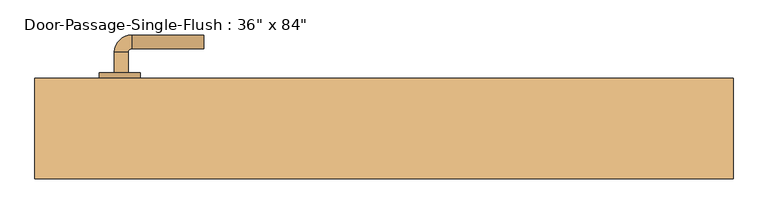
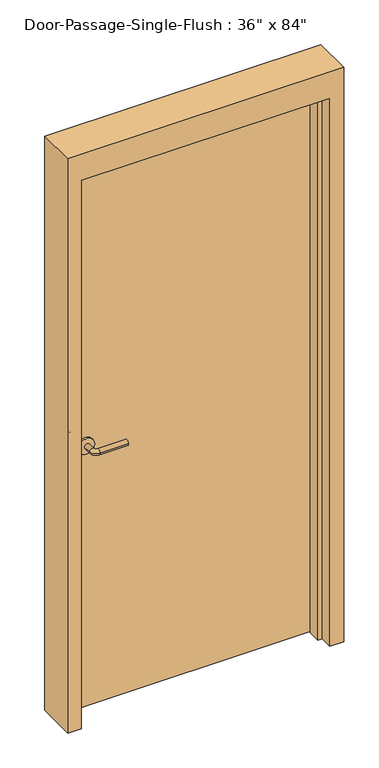
"""IFC4 building model written with IfcOpenShell, lengths in millimetres: door geometry."""

import ifcopenshell
import ifcopenshell.guid

model = None  # the IFC model being written
_history = None  # IfcOwnerHistory: only IFC2X3 demands one
_inside = {}  # id of a spatial element -> (the spatial element, [elements in it])
_under = {}  # id of a project, library or spatial element -> (it, [spatial elements below it])
_declared = {}  # id of a project -> (the project, [libraries it declares])
_typed = {}  # id of a type object -> (the type object, [elements of that type])
_made_of = {}  # id of a material, layer set ... -> (it, [elements and type objects made of it])


def new_model(schema):
    """Start an empty IFC model of exactly this schema.

    Asked for "IFC4X3", IfcOpenShell would pick the latest addendum, in which some entities
    have other attributes; the version numbers below select the first issue.
    IFC2X3 requires an IfcOwnerHistory on every rooted entity: one is made here for all.
    """
    global model, _history
    if schema == "IFC4X3":
        model = ifcopenshell.file(schema_version=(4, 3, 0, 0))
    else:
        model = ifcopenshell.file(schema=schema)
    _inside.clear()
    _under.clear()
    _declared.clear()
    _typed.clear()
    _made_of.clear()
    _history = None
    if model.schema == "IFC2X3":
        org = make("IfcOrganization", Name="unknown")
        user = make(
            "IfcPersonAndOrganization",
            ThePerson=make("IfcPerson", FamilyName="unknown"),
            TheOrganization=org,
        )
        app = make(
            "IfcApplication",
            ApplicationDeveloper=org,
            Version="unknown",
            ApplicationFullName="unknown",
            ApplicationIdentifier="unknown",
        )
        _history = make(
            "IfcOwnerHistory",
            OwningUser=user,
            OwningApplication=app,
            ChangeAction="ADDED",
            CreationDate=0,
        )
    return model


def make(cls, **values):
    """One entity of the class cls with the attributes given. An attribute that is None is left unset."""
    return model.create_entity(
        cls, **{name: value for name, value in values.items() if value is not None}
    )


def rooted(cls, **values):
    """An entity with a GlobalId (a new one), such as an element, a storey or a relation."""
    return make(cls, GlobalId=ifcopenshell.guid.new(), OwnerHistory=_history, **values)


def si_unit(unit_type, name, prefix=None):
    """IfcSIUnit, for example si_unit("LENGTHUNIT", "METRE", prefix="MILLI")."""
    return make("IfcSIUnit", UnitType=unit_type, Prefix=prefix, Name=name)


def assignment(units):
    """IfcUnitAssignment: the units of a project."""
    return None if units is None else make("IfcUnitAssignment", Units=units)


def point(xyz):
    """IfcCartesianPoint."""
    return None if xyz is None else make("IfcCartesianPoint", Coordinates=xyz)


def direction(xyz):
    """IfcDirection."""
    return None if xyz is None else make("IfcDirection", DirectionRatios=xyz)


def frame(location, z_axis=None, x_axis=None):
    """IfcAxis2Placement3D, a coordinate frame: its origin and axes. An axis left out is left unset."""
    return make(
        "IfcAxis2Placement3D",
        Location=point(location),
        Axis=direction(z_axis),
        RefDirection=direction(x_axis),
    )


def frame_2d(location, x_axis=None):
    """IfcAxis2Placement2D, a coordinate frame in the plane: its origin and x axis."""
    return make(
        "IfcAxis2Placement2D", Location=point(location), RefDirection=direction(x_axis)
    )


def origin():
    """The frame at (0, 0, 0) with its axes left unset."""
    return frame((0.0, 0.0, 0.0))


def origin_with_axes():
    """The frame at (0, 0, 0) with the z axis (0, 0, 1) and the x axis (1, 0, 0) written out."""
    return frame((0.0, 0.0, 0.0), z_axis=(0.0, 0.0, 1.0), x_axis=(1.0, 0.0, 0.0))


def place(relative_to, where):
    """IfcLocalPlacement: puts the frame where relative to a parent placement (None: the world)."""
    return make(
        "IfcLocalPlacement", PlacementRelTo=relative_to, RelativePlacement=where
    )


def context(
    kind, dimensions, precision=None, world=None, true_north=None, identifier=None
):
    """IfcGeometricRepresentationContext, for example the 3D "Model" context."""
    return make(
        "IfcGeometricRepresentationContext",
        ContextIdentifier=identifier,
        ContextType=kind,
        CoordinateSpaceDimension=dimensions,
        Precision=precision,
        WorldCoordinateSystem=world,
        TrueNorth=true_north,
    )


def project(units=None, contexts=None):
    """IfcProject with its units and contexts."""
    return rooted(
        "IfcProject",
        Name="project",
        RepresentationContexts=contexts,
        UnitsInContext=assignment(units),
    )


def spatial(cls, under=None, at=None, **own):
    """A site, building, storey or space (cls), placed at a placement, below another one or the project."""
    s = rooted(cls, ObjectPlacement=at, **own)
    if under is not None:
        _under.setdefault(under.id(), (under, []))[1].append(s)
    return s


def polyline(points):
    """IfcPolyline through the points."""
    return make("IfcPolyline", Points=[point(p) for p in points])


def circle_curve(where, radius):
    """IfcCircle in the frame where."""
    return make("IfcCircle", Position=where, Radius=radius)


def ellipse_curve(where, semi_axis1, semi_axis2):
    """IfcEllipse in the frame where."""
    return make(
        "IfcEllipse", Position=where, SemiAxis1=semi_axis1, SemiAxis2=semi_axis2
    )


def trimmed(basis, trim1, trim2, sense, master):
    """IfcTrimmedCurve: the piece of a basis curve between two trims."""
    return make(
        "IfcTrimmedCurve",
        BasisCurve=basis,
        Trim1=trim1,
        Trim2=trim2,
        SenseAgreement=sense,
        MasterRepresentation=master,
    )


def segment(curve, same_sense, transition):
    """IfcCompositeCurveSegment."""
    return make(
        "IfcCompositeCurveSegment",
        Transition=transition,
        SameSense=same_sense,
        ParentCurve=curve,
    )


def composite_curve(segments, self_intersect=None):
    """IfcCompositeCurve: segments joined end to end."""
    return make("IfcCompositeCurve", Segments=segments, SelfIntersect=self_intersect)


def outline(outer, holes=None, kind="AREA"):
    """IfcArbitraryClosedProfileDef: a profile drawn as a closed curve; with holes, ...WithVoids."""
    if holes is None:
        return make("IfcArbitraryClosedProfileDef", ProfileType=kind, OuterCurve=outer)
    return make(
        "IfcArbitraryProfileDefWithVoids",
        ProfileType=kind,
        OuterCurve=outer,
        InnerCurves=holes,
    )


def extrude(swept, where, along, depth):
    """IfcExtrudedAreaSolid: the profile swept, set in the frame where, extruded along a direction by depth."""
    return make(
        "IfcExtrudedAreaSolid",
        SweptArea=swept,
        Position=where,
        ExtrudedDirection=direction(along),
        Depth=depth,
    )


def faces_of(points, faces, orient=None, outer=None):
    """IfcFace entities. A face is a list of loops; a loop is a list of indices into points, from 0.

    orient and outer hold one flag for each loop. By default every Orientation is true, the
    first loop of a face is its IfcFaceOuterBound and the others are IfcFaceBound.
    """
    made = []
    for i, loops in enumerate(faces):
        bounds = []
        for j, loop in enumerate(loops):
            is_outer = j == 0 if outer is None else outer[i][j]
            bounds.append(
                make(
                    "IfcFaceOuterBound" if is_outer else "IfcFaceBound",
                    Bound=make("IfcPolyLoop", Polygon=[points[k] for k in loop]),
                    Orientation=True if orient is None else orient[i][j],
                )
            )
        made.append(make("IfcFace", Bounds=bounds))
    return made


def faceted_brep(points, faces, orient=None, outer=None, voids=None):
    """IfcFacetedBrep: a solid bounded by flat faces; with voids (closed shells), ...WithVoids."""
    shared = [point(p) for p in points]
    hull = make("IfcClosedShell", CfsFaces=faces_of(shared, faces, orient, outer))
    if voids is None:
        return make("IfcFacetedBrep", Outer=hull)
    return make(
        "IfcFacetedBrepWithVoids",
        Outer=hull,
        Voids=[
            make(cls, CfsFaces=faces_of(shared, fs, o, b)) for cls, fs, o, b in voids
        ],
    )


def shape(context_of_items, identifier, shape_type, items):
    """IfcShapeRepresentation: the items that make up one representation, for example the "Body"."""
    return make(
        "IfcShapeRepresentation",
        ContextOfItems=context_of_items,
        RepresentationIdentifier=identifier,
        RepresentationType=shape_type,
        Items=items,
    )


def source(mapping_origin, context_of_items, identifier, shape_type, items):
    """IfcRepresentationMap: a shape defined once, which mapped items show again and again."""
    return make(
        "IfcRepresentationMap",
        MappingOrigin=mapping_origin,
        MappedRepresentation=shape(context_of_items, identifier, shape_type, items),
    )


def transform(
    local_origin,
    x_axis=None,
    y_axis=None,
    z_axis=None,
    scale=None,
    scale2=None,
    scale3=None,
    uniform=True,
):
    """IfcCartesianTransformationOperator3D, or its non-uniform kind. x_axis, y_axis, z_axis: its Axis1, 2, 3."""
    if uniform:
        return make(
            "IfcCartesianTransformationOperator3D",
            Axis1=direction(x_axis),
            Axis2=direction(y_axis),
            LocalOrigin=point(local_origin),
            Scale=scale,
            Axis3=direction(z_axis),
        )
    return make(
        "IfcCartesianTransformationOperator3DnonUniform",
        Axis1=direction(x_axis),
        Axis2=direction(y_axis),
        LocalOrigin=point(local_origin),
        Scale=scale,
        Axis3=direction(z_axis),
        Scale2=scale2,
        Scale3=scale3,
    )


def mapped(mapping_source, mapping_target):
    """IfcMappedItem: shows the shape of a source again, moved by a transform."""
    return make(
        "IfcMappedItem", MappingSource=mapping_source, MappingTarget=mapping_target
    )


def made_of(thing, what):
    """Note that an element or type object is made of a material, layer set ...; save() writes the relation."""
    if what is not None:
        _made_of.setdefault(what.id(), (what, []))[1].append(thing)
    return thing


def element(
    cls,
    number,
    at=None,
    inside=None,
    cuts=None,
    type_object=None,
    material=None,
    context=None,
    identifier="Body",
    shape_type=None,
    held_by="IfcProductDefinitionShape",
    body=None,
    shapes=None,
    **own,
):
    """One element of the class cls, such as IfcWall. Its Tag is "e" and its number.

    at: its placement. inside: the storey or other place that contains it. cuts: it is an
    opening in that element (IfcRelVoidsElement). A single representation is given by context,
    identifier, shape_type and body (its items); several are given by shapes. held_by: the class
    of the entity that holds the representations. save() writes the other relations.
    """
    e = rooted(cls, Tag="e%d" % number, ObjectPlacement=at, **own)
    if body is not None:
        shapes = [shape(context, identifier, shape_type, body)]
    if shapes is not None:
        e.Representation = make(held_by, Representations=shapes)
    if inside is not None:
        _inside.setdefault(inside.id(), (inside, []))[1].append(e)
    if cuts is not None:
        rooted(
            "IfcRelVoidsElement", RelatingBuildingElement=cuts, RelatedOpeningElement=e
        )
    if type_object is not None:
        _typed.setdefault(type_object.id(), (type_object, []))[1].append(e)
    return made_of(e, material)


def aggregate(whole, parts):
    """IfcRelAggregates: a whole, such as a stair, and the parts it consists of."""
    return rooted("IfcRelAggregates", RelatingObject=whole, RelatedObjects=parts)


def save(model, path):
    """Write the relations noted so far, then the file.

    IfcRelAggregates (storeys below a building ...), IfcRelContainedInSpatialStructure (elements
    in a storey), IfcRelDefinesByType, IfcRelAssociatesMaterial and IfcRelDeclares: one each for
    every whole, place, type object, material and project.
    """
    for whole, parts in _under.values():
        aggregate(whole, parts)
    for where, things in _inside.values():
        rooted(
            "IfcRelContainedInSpatialStructure",
            RelatedElements=things,
            RelatingStructure=where,
        )
    for kind, things in _typed.values():
        rooted("IfcRelDefinesByType", RelatedObjects=things, RelatingType=kind)
    for what, things in _made_of.values():
        rooted("IfcRelAssociatesMaterial", RelatedObjects=things, RelatingMaterial=what)
    for by, libraries in _declared.values():
        rooted("IfcRelDeclares", RelatingContext=by, RelatedDefinitions=libraries)
    model.write(path)


def plane_surface(at):
    """IfcPlane: the flat surface through the origin of the frame at, square to its z axis."""
    return make("IfcPlane", Position=at)


def cylinder_surface(at, radius):
    """IfcCylindricalSurface: all points at the distance radius from the z axis of the frame at."""
    return make("IfcCylindricalSurface", Position=at, Radius=radius)


def revolved_surface(curve, axis_point, axis_direction):
    """IfcSurfaceOfRevolution: the curve turned about the line through axis_point along axis_direction."""
    return make(
        "IfcSurfaceOfRevolution",
        SweptCurve=make("IfcArbitraryOpenProfileDef", ProfileType="CURVE", Curve=curve),
        AxisPosition=make("IfcAxis1Placement", Location=point(axis_point), Axis=direction(axis_direction)),
    )


def advanced_brep(points, edges, surfaces, faces):
    """IfcAdvancedBrep: a solid bounded by faces that lie on surfaces and meet in shared edges.

    An edge is (start, end): straight between two places in points (the first is 0);
    or (start, end, curve); or (start, end, curve, False) where it runs against its curve.
    A face is (place in surfaces, loops), or (place, loops, False) where it looks against
    its surface's normal. A loop lists edges by number (the first is 1), with a minus sign
    where the edge is run from its end to its start. The first loop is the outer one.
    """
    corners = [point(p) for p in points]
    vertices = [make("IfcVertexPoint", VertexGeometry=c) for c in corners]
    made = []
    for start, end, *more in edges:
        made.append(
            make(
                "IfcEdgeCurve",
                EdgeStart=vertices[start],
                EdgeEnd=vertices[end],
                EdgeGeometry=more[0] if more else make("IfcPolyline", Points=[corners[start], corners[end]]),
                SameSense=more[1] if len(more) > 1 else True,
            )
        )
    hull = []
    for where, loops, *sense in faces:
        bounds = []
        for j, loop in enumerate(loops):
            ring = [make("IfcOrientedEdge", EdgeElement=made[abs(k) - 1], Orientation=k > 0) for k in loop]
            bounds.append(
                make(
                    "IfcFaceOuterBound" if j == 0 else "IfcFaceBound",
                    Bound=make("IfcEdgeLoop", EdgeList=ring),
                    Orientation=True,
                )
            )
        hull.append(make("IfcAdvancedFace", Bounds=bounds, FaceSurface=surfaces[where], SameSense=sense[0] if sense else True))
    return make("IfcAdvancedBrep", Outer=make("IfcClosedShell", CfsFaces=hull))


def door_a8315dbd(model_context):
    return source(origin(), model_context, "Body", "SolidModel", [
        advanced_brep(
        [(-392.190625, 15.8125, 1016.0), (-372.190625, 15.8125, 1016.0), (-372.190625, -14.1875, 1016.0), (-392.190625, -14.1875, 1016.0), (-367.190625, -19.1875, 1016.0), (-367.190625, -39.1875, 1016.0), (-262.190625, -39.1875, 1016.0), (-262.190625, -19.1875, 1016.0)],
        [
            (0, 1, circle_curve(frame((-382.190625, 15.8125, 1016.0), z_axis=(0.0, 1.0, 0.0), x_axis=(1.0, 0.0, 0.0)), 10.0)),
            (1, 0, circle_curve(frame((-382.190625, 15.8125, 1016.0), z_axis=(0.0, 1.0, 0.0), x_axis=(1.0, 0.0, 0.0)), 10.0)),
            (1, 2),
            (2, 3, circle_curve(frame((-382.190625, -14.1875, 1016.0), z_axis=(0.0, 1.0, 0.0), x_axis=(1.0, 0.0, 0.0)), 10.0)),
            (3, 0),
            (3, 2, circle_curve(frame((-382.190625, -14.1875, 1016.0), z_axis=(0.0, 1.0, 0.0), x_axis=(1.0, 0.0, 0.0)), 10.0)),
            (4, 5, circle_curve(frame((-367.190625, -29.1875, 1016.0), z_axis=(-1.0, 0.0, 0.0), x_axis=(0.0, 1.0, 0.0)), 10.0)),
            (5, 3, circle_curve(frame((-367.190625, -14.1875, 1016.0), z_axis=(0.0, 0.0, -1.0), x_axis=(-1.0, 0.0, 0.0)), 25.0)),
            (2, 4, circle_curve(frame((-367.190625, -14.1875, 1016.0), z_axis=(0.0, 0.0, 1.0), x_axis=(-1.0, 0.0, 0.0)), 5.0)),
            (5, 4, circle_curve(frame((-367.190625, -29.1875, 1016.0), z_axis=(-1.0, 0.0, 0.0), x_axis=(0.0, 1.0, 0.0)), 10.0)),
            (6, 7, circle_curve(frame((-262.190625, -29.1875, 1016.0), z_axis=(1.0, 0.0, 0.0), x_axis=(0.0, 1.0, 0.0)), 10.0)),
            (7, 6, circle_curve(frame((-262.190625, -29.1875, 1016.0), z_axis=(1.0, 0.0, 0.0), x_axis=(0.0, 1.0, 0.0)), 10.0)),
            (4, 7),
            (6, 5),
        ],
        [
            plane_surface(frame((-382.190625, 15.8125, 1016.0), z_axis=(0.0, 1.0, 0.0), x_axis=(0.0, 0.0, 1.0))),
            cylinder_surface(frame((-382.190625, 15.8125, 1016.0), z_axis=(0.0, 1.0, 0.0), x_axis=(1.0, 0.0, 0.0)), 10.0),
            revolved_surface(trimmed(ellipse_curve(frame((-382.190625, -14.1875, 1016.0), z_axis=(0.0, -1.0, 0.0), x_axis=(1.0, 0.0, 0.0)), 10.0, 10.0), [point((-392.190625, -14.1875, 1016.0))], [point((-372.190625, -14.1875, 1016.0))], True, "CARTESIAN"), (-367.190625, -14.1875, 1016.0), (0.0, 0.0, -1.0)),
            revolved_surface(trimmed(ellipse_curve(frame((-382.190625, -14.1875, 1016.0), z_axis=(0.0, -1.0, 0.0), x_axis=(1.0, 0.0, 0.0)), 10.0, 10.0), [point((-372.190625, -14.1875, 1016.0))], [point((-392.190625, -14.1875, 1016.0))], True, "CARTESIAN"), (-367.190625, -14.1875, 1016.0), (0.0, 0.0, -1.0)),
            plane_surface(frame((-262.190625, -29.1875, 1016.0), z_axis=(1.0, 0.0, 0.0), x_axis=(0.0, 0.0, 1.0))),
            cylinder_surface(frame((-367.190625, -29.1875, 1016.0), z_axis=(-1.0, 0.0, 0.0), x_axis=(0.0, 1.0, 0.0)), 10.0),
        ],
        [
            (0, [[1, 2]]),
            (1, [[3, 4, 5, -2]]),
            (1, [[-5, 6, -3, -1]]),
            (2, [[7, 8, -4, 9]]),
            (3, [[10, -9, -6, -8]]),
            (4, [[11, 12]]),
            (5, [[13, -11, 14, -7]]),
            (5, [[-14, -12, -13, -10]]),
        ],
    ),
        extrude(outline(composite_curve([segment(trimmed(circle_curve(frame_2d((1016.0, -384.690625)), 30.0), [point((1016.0, -414.690625))], [point((1016.0, -354.690625))], False, "CARTESIAN"), True, "CONTINUOUS"), segment(trimmed(circle_curve(frame_2d((1016.0, -384.690625)), 30.0), [point((1016.0, -354.690625))], [point((1016.0, -414.690625))], False, "CARTESIAN"), True, "CONTINUOUS")], self_intersect=False)), frame((0.0, 15.8125, 0.0), z_axis=(0.0, 1.0, 0.0), x_axis=(0.0, 0.0, 1.0)), (0.0, 0.0, 1.0), 8.0),
        advanced_brep(
        [(-392.190625, 76.2625, 1016.0), (-372.190625, 76.2625, 1016.0), (-392.190625, 106.2625, 1016.0), (-372.190625, 106.2625, 1016.0), (-367.190625, 111.2625, 1016.0), (-367.190625, 131.2625, 1016.0), (-262.190625, 131.2625, 1016.0), (-262.190625, 111.2625, 1016.0)],
        [
            (0, 1, circle_curve(frame((-382.190625, 76.2625, 1016.0), z_axis=(0.0, -1.0, 0.0), x_axis=(1.0, 0.0, 0.0)), 10.0)),
            (1, 0, circle_curve(frame((-382.190625, 76.2625, 1016.0), z_axis=(0.0, -1.0, 0.0), x_axis=(1.0, 0.0, 0.0)), 10.0)),
            (0, 2),
            (2, 3, circle_curve(frame((-382.190625, 106.2625, 1016.0), z_axis=(0.0, -1.0, 0.0), x_axis=(1.0, 0.0, 0.0)), 10.0)),
            (3, 1),
            (3, 2, circle_curve(frame((-382.190625, 106.2625, 1016.0), z_axis=(0.0, -1.0, 0.0), x_axis=(1.0, 0.0, 0.0)), 10.0)),
            (4, 3, circle_curve(frame((-367.190625, 106.2625, 1016.0), z_axis=(0.0, 0.0, 1.0), x_axis=(-1.0, 0.0, 0.0)), 5.0)),
            (2, 5, circle_curve(frame((-367.190625, 106.2625, 1016.0), z_axis=(0.0, 0.0, -1.0), x_axis=(-1.0, 0.0, 0.0)), 25.0)),
            (5, 4, circle_curve(frame((-367.190625, 121.2625, 1016.0), z_axis=(-1.0, 0.0, 0.0), x_axis=(0.0, -1.0, 0.0)), 10.0)),
            (4, 5, circle_curve(frame((-367.190625, 121.2625, 1016.0), z_axis=(-1.0, 0.0, 0.0), x_axis=(0.0, -1.0, 0.0)), 10.0)),
            (6, 7, circle_curve(frame((-262.190625, 121.2625, 1016.0), z_axis=(1.0, 0.0, 0.0), x_axis=(0.0, -1.0, 0.0)), 10.0)),
            (7, 6, circle_curve(frame((-262.190625, 121.2625, 1016.0), z_axis=(1.0, 0.0, 0.0), x_axis=(0.0, -1.0, 0.0)), 10.0)),
            (5, 6),
            (7, 4),
        ],
        [
            plane_surface(frame((-382.190625, 76.2625, 1016.0), z_axis=(0.0, -1.0, 0.0), x_axis=(0.0, 0.0, 1.0))),
            cylinder_surface(frame((-382.190625, 76.2625, 1016.0), z_axis=(0.0, -1.0, 0.0), x_axis=(1.0, 0.0, 0.0)), 10.0),
            revolved_surface(trimmed(ellipse_curve(frame((-382.190625, 106.2625, 1016.0), z_axis=(0.0, -1.0, 0.0), x_axis=(1.0, 0.0, 0.0)), 10.0, 10.0), [point((-392.190625, 106.2625, 1016.0))], [point((-372.190625, 106.2625, 1016.0))], True, "CARTESIAN"), (-367.190625, 106.2625, 1016.0), (0.0, 0.0, -1.0)),
            revolved_surface(trimmed(ellipse_curve(frame((-382.190625, 106.2625, 1016.0), z_axis=(0.0, -1.0, 0.0), x_axis=(1.0, 0.0, 0.0)), 10.0, 10.0), [point((-372.190625, 106.2625, 1016.0))], [point((-392.190625, 106.2625, 1016.0))], True, "CARTESIAN"), (-367.190625, 106.2625, 1016.0), (0.0, 0.0, -1.0)),
            plane_surface(frame((-262.190625, 121.2625, 1016.0), z_axis=(1.0, 0.0, 0.0), x_axis=(0.0, 0.0, 1.0))),
            cylinder_surface(frame((-367.190625, 121.2625, 1016.0), z_axis=(-1.0, 0.0, 0.0), x_axis=(0.0, -1.0, 0.0)), 10.0),
        ],
        [
            (0, [[1, 2]]),
            (1, [[-1, 3, 4, 5]]),
            (1, [[-2, -5, 6, -3]]),
            (2, [[7, -4, 8, 9]]),
            (3, [[-8, -6, -7, 10]]),
            (4, [[11, 12]]),
            (5, [[-9, 13, -12, 14]]),
            (5, [[-10, -14, -11, -13]]),
        ],
    ),
        extrude(outline(composite_curve([segment(trimmed(circle_curve(frame_2d((1016.0, -384.690625)), 30.0), [point((1016.0, -414.690625))], [point((1016.0, -354.690625))], False, "CARTESIAN"), True, "CONTINUOUS"), segment(trimmed(circle_curve(frame_2d((1016.0, -384.690625)), 30.0), [point((1016.0, -354.690625))], [point((1016.0, -414.690625))], False, "CARTESIAN"), True, "CONTINUOUS")], self_intersect=False)), frame((0.0, 68.2625, 0.0), z_axis=(0.0, 1.0, 0.0), x_axis=(0.0, 0.0, 1.0)), (0.0, 0.0, 1.0), 8.0),
        faceted_brep([(457.2, 19.05, 0.0), (457.2, 68.2625, 0.0), (508.0, 68.2625, 0.0), (508.0, -77.7875, 0.0), (457.2, -77.7875, 0.0), (457.2, -28.575, 0.0), (441.325, -28.575, 0.0), (441.325, 19.05, 0.0), (457.2, 19.05, 2133.6), (457.2, 68.2625, 2133.6), (-457.2, 68.2625, 2133.6), (-457.2, 68.2625, 0.0), (-508.0, 68.2625, 0.0), (-508.0, 68.2625, 2235.2), (508.0, 68.2625, 2235.2), (508.0, -77.7875, 2235.2), (-508.0, -77.7875, 2235.2), (-508.0, -77.7875, 0.0), (-457.2, -77.7875, 0.0), (-457.2, -77.7875, 2133.6), (457.2, -77.7875, 2133.6), (457.2, -28.575, 2133.6), (-457.2, -28.575, 2133.6), (-457.2, -28.575, 0.0), (-441.325, -28.575, 0.0), (-441.325, -28.575, 2117.725), (441.325, -28.575, 2117.725), (441.325, 19.05, 2117.725), (-441.325, 19.05, 2117.725), (-441.325, 19.05, 0.0), (-457.2, 19.05, 0.0), (-457.2, 19.05, 2133.6)], [[[0, 1, 2, 3, 4, 5, 6, 7]], [[1, 0, 8, 9]], [[2, 1, 9, 10, 11, 12, 13, 14]], [[3, 2, 14, 15]], [[4, 3, 15, 16, 17, 18, 19, 20]], [[5, 4, 20, 21]], [[6, 5, 21, 22, 23, 24, 25, 26]], [[7, 6, 26, 27]], [[0, 7, 27, 28, 29, 30, 31, 8]], [[9, 8, 31, 10]], [[20, 19, 22, 21]], [[26, 25, 28, 27]], [[12, 11, 30, 29, 24, 23, 18, 17]], [[11, 10, 31, 30]], [[13, 12, 17, 16]], [[19, 18, 23, 22]], [[25, 24, 29, 28]], [[15, 14, 13, 16]]]),
        extrude(outline(polyline([(457.2, 23.8125), (-457.2, 23.8125), (-457.2, 68.2625), (457.2, 68.2625), (457.2, 23.8125)])), origin_with_axes(), (0.0, 0.0, 1.0), 2133.6),
    ])


if __name__ == "__main__":
    model = new_model("IFC4")
    model_context = context("Model", 3, world=origin())
    ifc_project = project(units=[si_unit("LENGTHUNIT", "METRE", prefix="MILLI")], contexts=[model_context])
    site = spatial("IfcSite", under=ifc_project)
    building = spatial("IfcBuilding", under=site)
    placement = place(None, origin())
    door_shape = door_a8315dbd(model_context)
    element("IfcDoor", 1, ObjectType="Door-Passage-Single-Flush : 36\" x 84\"", at=placement, inside=building, context=model_context, shape_type="MappedRepresentation", body=[
        mapped(door_shape, transform((0.0, 0.0, 0.0), x_axis=(1.0, 0.0, 0.0), y_axis=(0.0, 1.0, 0.0), z_axis=(0.0, 0.0, 1.0))),
    ])
    save(model, "model.ifc")

# Revit data of these elements
# Type "Door-Passage-Single-Flush : 36\" x 84\""
#   Type Mark = "35"
#   Assembly Code = "B2030200"
#   Analytic Construction = "Wooden"
#   Thickness = 0' - 1 3/4"
#   Thermal Resistance (R) = 2.5876 (h·ft²·°F)/BTU
#   Swing Angle [instance default] = 90.00°
#   Strike Height = 3' - 4"
#   Rough Width [instance default] = 3' - 4"
#   Rough Height [instance default] = 7' - 4"
#   MF Opening Height [instance default] = 0' - 4"
#   MF Opening Width [instance default] = 0' - 4"
#   Inset Calculate [instance default] = 0' - 4"
#   Masonry Inset [instance default] = 0' - 1"
#   Height = 7' - 0"
#   Width = 3' - 0"
#   Heat Transfer Coefficient (U) = 0.3865 BTU/(h·ft²·°F)
#   Masonry Frame Depth = 0' - 5 3/4"
#   Masonry Frame [instance default] = yes
#   Function = 1
#   Dry Wall Frame [instance default] = no
#   Panel Material = Wood - Birch
#   Frame Material = Metal - Paint Finish - Grey
#   Door Handle Material = Aluminum
#   Visual Light Transmittance = 0
#   Solar Heat Gain Coefficient = 0
#   Wall Closure = (empty or 0)
# Element 1 (IfcDoor, "Door-Passage-Single-Flush : 36\" x 84\"")
#   Inset Calculate = 0' - 3"
#   Masonry Inset = 0' - 0"
#   Materials on its faces: "Aluminum", "Metal - Paint Finish - Grey", "Wood - Birch"
# Materials
#   "Wood - Birch": class "Wood", colour RGB 166 116 52, transparency 0, Cost = 0
#   "Metal - Paint Finish - Grey": class "Paint", colour RGB 104 104 104, transparency 0, Cost = 0
#   "Aluminum": class "Metal", colour RGB 247 247 247, transparency 0, Description = "Aluminum 6061", Cost = 0
